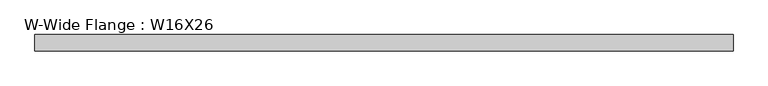
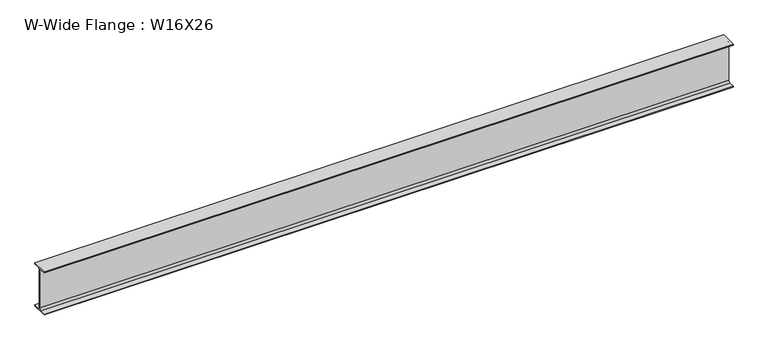
"""IFC4 building model written with IfcOpenShell, lengths in millimetres: beam geometry, W-Wide Flange : W16X26."""

from ifc_helpers import new_model, si_unit, point, frame, frame_2d, origin, place, context, project, spatial, polyline, circle_curve, trimmed, segment, composite_curve, outline, extrude, source, transform, mapped, element, save


def w_wide_flange_w16x26_42a353e8(model_context):
    return source(origin(), model_context, "Body", "SweptSolid", [
        extrude(outline(composite_curve([segment(polyline([(69.85, -190.627), (69.85, -199.39), (-69.85, -199.39), (-69.85, -190.627), (-21.3995, -190.627)]), True, "CONTINUOUS"), segment(trimmed(circle_curve(frame_2d((-21.3995, -172.4025)), 18.2245), [point((-21.3995, -190.627))], [point((-3.175, -172.4025))], True, "CARTESIAN"), True, "CONTINUOUS"), segment(polyline([(-3.175, -172.4025), (-3.175, 172.4025)]), True, "CONTINUOUS"), segment(trimmed(circle_curve(frame_2d((-21.3995, 172.4025)), 18.2245), [point((-3.175, 172.4025))], [point((-21.3995, 190.627))], True, "CARTESIAN"), True, "CONTINUOUS"), segment(polyline([(-21.3995, 190.627), (-69.85, 190.627), (-69.85, 199.39), (69.85, 199.39), (69.85, 190.627), (21.3995, 190.627)]), True, "CONTINUOUS"), segment(trimmed(circle_curve(frame_2d((21.3995, 172.4025)), 18.2245), [point((21.3995, 190.627))], [point((3.175, 172.4025))], True, "CARTESIAN"), True, "CONTINUOUS"), segment(polyline([(3.175, 172.4025), (3.175, -172.4025)]), True, "CONTINUOUS"), segment(trimmed(circle_curve(frame_2d((21.3995, -172.4025)), 18.2245), [point((3.175, -172.4025))], [point((21.3995, -190.627))], True, "CARTESIAN"), True, "CONTINUOUS"), segment(polyline([(21.3995, -190.627), (69.85, -190.627)]), True, "CONTINUOUS")], self_intersect=False)), frame((-3016.8063621, 0.0, 0.0), z_axis=(1.0, 0.0, 0.0), x_axis=(0.0, 1.0, 0.0)), (0.0, 0.0, 1.0), 6012.7527361),
    ])


if __name__ == "__main__":
    model = new_model("IFC4")
    model_context = context("Model", 3, world=origin())
    ifc_project = project(units=[si_unit("LENGTHUNIT", "METRE", prefix="MILLI")], contexts=[model_context])
    site = spatial("IfcSite", under=ifc_project)
    building = spatial("IfcBuilding", under=site)
    placement = place(None, origin())
    w_wide_flange_w16x26_shape = w_wide_flange_w16x26_42a353e8(model_context)
    element("IfcBeam", 1, ObjectType="W-Wide Flange : W16X26", at=placement, inside=building, context=model_context, shape_type="MappedRepresentation", body=[
        mapped(w_wide_flange_w16x26_shape, transform((0.0, 0.0, 0.0), x_axis=(1.0, 0.0, 0.0), y_axis=(0.0, 1.0, 0.0), z_axis=(0.0, 0.0, 1.0))),
    ])
    save(model, "model.ifc")

# Revit data of these elements
# Type "W-Wide Flange : W16X26"
#   Assembly Code = "B10"
#   W = 26
#   Length [instance default] = 5' - 0"
#   bf = 0' - 5 1/2"
#   d = 1' - 3.7"
#   k = 0' - 1 1/16"
#   k2 = 0' - 0.7175"
#   tf = 0' - 0.345"
#   tw = 0' - 0 1/4"
#   A = 0.0533333 SF
#   Structural Material [instance default] = Steel ASTM A992
# Element 1 (IfcBeam, "W-Wide Flange : W16X26")
#   Structural Material = Steel ASTM A36
#   Materials on its faces: "Steel ASTM A36"
# Materials
#   "Steel ASTM A992": class "Metal", colour RGB 199 199 199, transparency 0, Description = "Structural steel 50ksi", Cost = 0
#   "Steel ASTM A36": class "Metal", colour RGB 199 199 199, transparency 0, Description = "Structural steel, ASTM A36 Grade B, mill finish", Cost = 0
